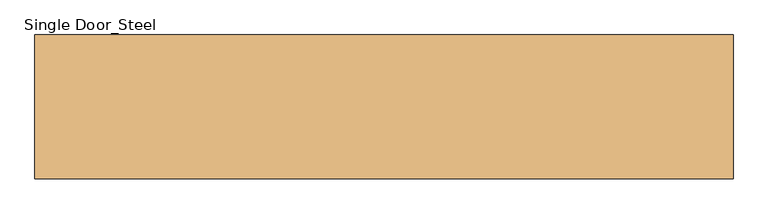
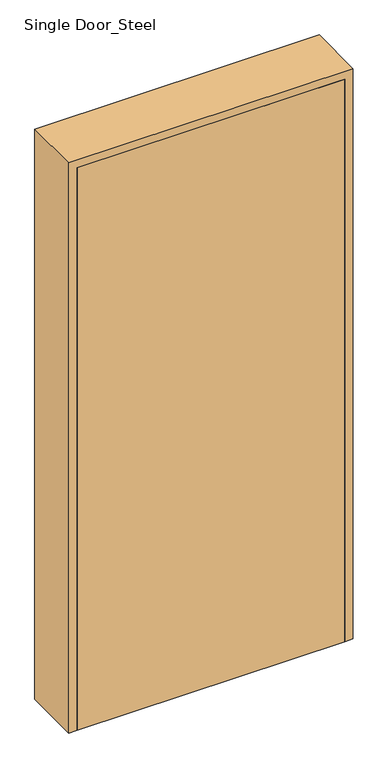
"""IFC4 building model written with IfcOpenShell, lengths in millimetres: door geometry, Single Door_Steel : H_DR_AR B12_Door_Single FSD 01."""

from ifc_helpers import new_model, si_unit, origin, origin_with_axes, place, context, project, spatial, polyline, outline, extrude, faceted_brep, source, transform, mapped, element, save


def single_door_steel_b319cbd1(model_context):
    return source(origin(), model_context, "Body", "SolidModel", [
        extrude(outline(polyline([(480.0, -105.0), (-480.0, -105.0), (-480.0, -70.0), (480.0, -70.0), (480.0, -105.0)])), origin_with_axes(), (0.0, 0.0, 1.0), 2130.0),
        faceted_brep([(480.0, -105.0, 0.0), (480.0, -70.0, 0.0), (460.0, -70.0, 0.0), (460.0, 70.0, 0.0), (480.0, 70.0, 0.0), (480.0, 105.0, 0.0), (510.0, 105.0, 0.0), (510.0, -105.0, 0.0), (510.0, -105.0, 2160.0), (-510.0, -105.0, 2160.0), (-510.0, -105.0, 0.0), (-480.0, -105.0, 0.0), (-480.0, -105.0, 2130.0), (480.0, -105.0, 2130.0), (510.0, 105.0, 2160.0), (480.0, 105.0, 2130.0), (-480.0, 105.0, 2130.0), (-480.0, 105.0, 0.0), (-510.0, 105.0, 0.0), (-510.0, 105.0, 2160.0), (480.0, 70.0, 2130.0), (460.0, 70.0, 2110.0), (-460.0, 70.0, 2110.0), (-460.0, 70.0, 0.0), (-480.0, 70.0, 0.0), (-480.0, 70.0, 2130.0), (460.0, -70.0, 2110.0), (480.0, -70.0, 2130.0), (-480.0, -70.0, 2130.0), (-480.0, -70.0, 0.0), (-460.0, -70.0, 0.0), (-460.0, -70.0, 2110.0)], [[[0, 1, 2, 3, 4, 5, 6, 7]], [[7, 8, 9, 10, 11, 12, 13, 0]], [[6, 14, 8, 7]], [[5, 15, 16, 17, 18, 19, 14, 6]], [[4, 20, 15, 5]], [[3, 21, 22, 23, 24, 25, 20, 4]], [[2, 26, 21, 3]], [[1, 27, 28, 29, 30, 31, 26, 2]], [[0, 13, 27, 1]], [[12, 11, 29, 28]], [[11, 10, 18, 17, 24, 23, 30, 29]], [[19, 18, 10, 9]], [[25, 24, 17, 16]], [[31, 30, 23, 22]], [[14, 19, 9, 8]], [[20, 25, 16, 15]], [[26, 31, 22, 21]], [[13, 12, 28, 27]]]),
    ])


if __name__ == "__main__":
    model = new_model("IFC4")
    model_context = context("Model", 3, world=origin())
    ifc_project = project(units=[si_unit("LENGTHUNIT", "METRE", prefix="MILLI")], contexts=[model_context])
    site = spatial("IfcSite", under=ifc_project)
    building = spatial("IfcBuilding", under=site)
    placement = place(None, origin())
    single_door_steel_shape = single_door_steel_b319cbd1(model_context)
    element("IfcDoor", 1, ObjectType="Single Door_Steel : H_DR_AR B12_Door_Single FSD 01", at=placement, inside=building, context=model_context, shape_type="MappedRepresentation", body=[
        mapped(single_door_steel_shape, transform((0.0, 0.0, 0.0), x_axis=(1.0, 0.0, 0.0), y_axis=(0.0, 1.0, 0.0), z_axis=(0.0, 0.0, 1.0))),
    ])
    save(model, "model.ifc")

# Revit data of these elements
# Type "Single Door_Steel : H_DR_AR B12_Door_Single FSD 01"
#   Type Mark = "FRD"
#   Analytic Construction = "<None>"
#   프레임 투영 외부. = 25 mm
#   프레임 투영 내부. = 25 mm
#   프레임 폭 = 75 mm
#   Height = 2160 mm
#   Width = 1020 mm
#   Define Thermal Properties by = 1
#   문 패널 = none
#   문 프레임 = none
#   Function = (empty or 0)
#   Wall Closure = (empty or 0)
